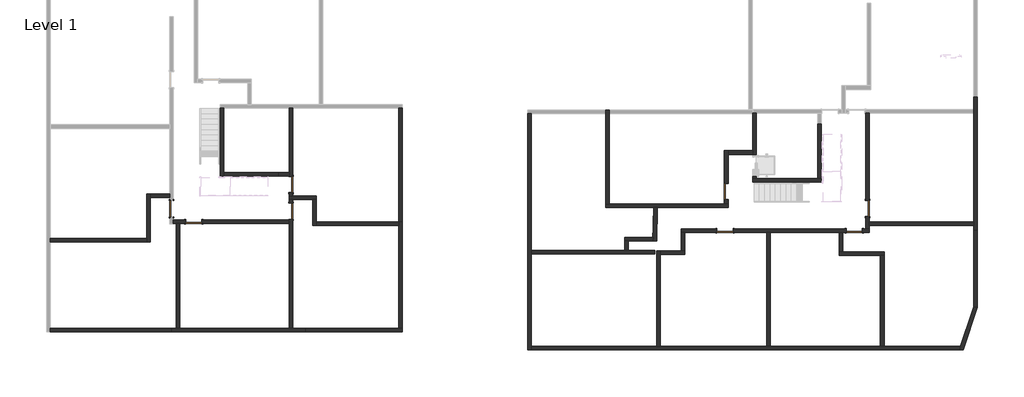
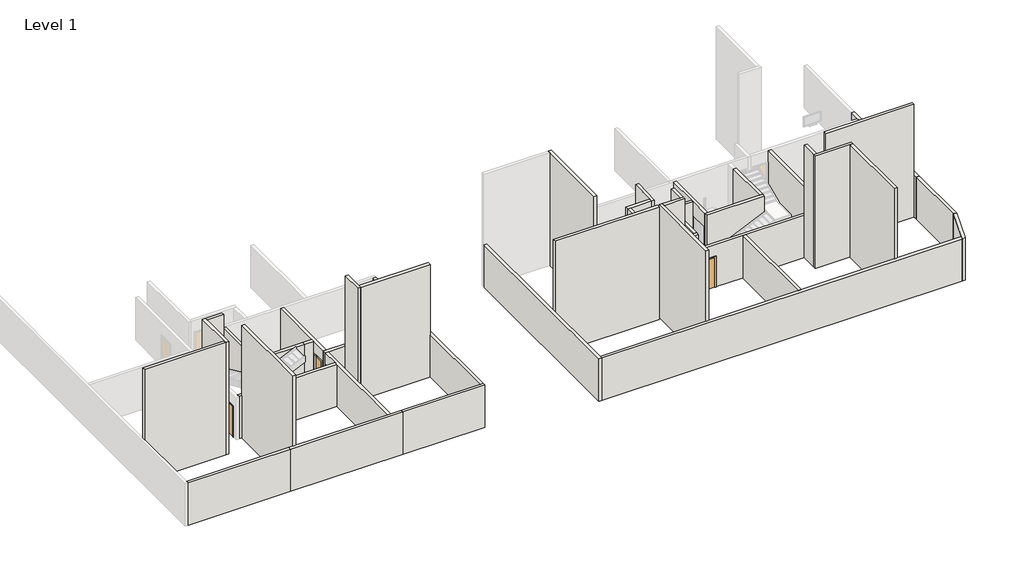
# One storey, part 1 of 2: 44 walls, 8 doors.
# Revit data of these elements (continued)
# Room, not placed, phase "New Construction", upper offset 0 cm, lower offset 0 cm
#   Number = "5"
#   Name = "Room"
# Room, not placed, phase "New Construction", upper offset 0 cm, lower offset 0 cm
#   Number = "6"
#   Name = "Room"
# Room at (-9476.825, 5160.6) mm, phase "New Construction", upper level "Level 1", upper offset 243.84 cm, lower offset 0 cm
#   Number = "124"
#   Name = "Room"
# Room, not placed, phase "New Construction", upper offset 0 cm, lower offset 0 cm
#   Number = "34"
#   Name = "Room"
# Room, not placed, phase "New Construction", upper offset 0 cm, lower offset 0 cm
#   Number = "35"
#   Name = "Room"
# Room, not placed, phase "New Construction", upper offset 0 cm, lower offset 0 cm
#   Number = "9"
#   Name = "Room"
# Room, not placed, phase "New Construction", upper offset 0 cm, lower offset 0 cm
#   Number = "10"
#   Name = "Room"
# Room, not placed, phase "New Construction", upper offset 0 cm, lower offset 0 cm
#   Number = "125"
#   Name = "Room"
# Room, not placed, phase "New Construction", upper offset 0 cm, lower offset 0 cm
#   Number = "126"
#   Name = "Room"
# Room, not placed, phase "New Construction", upper offset 0 cm, lower offset 0 cm
#   Number = "127"
#   Name = "Room"
# Room, not placed, phase "New Construction", upper offset 0 cm, lower offset 0 cm
#   Number = "128"
#   Name = "Room"
# Room, not placed, phase "New Construction", upper offset 0 cm, lower offset 0 cm
#   Number = "129"
#   Name = "Room"
# Room, not placed, phase "New Construction", upper offset 0 cm, lower offset 0 cm
#   Number = "91"
#   Name = "Room"
# Room at (-20321.225, 11202.195) mm, phase "New Construction", upper level "Level 1", upper offset 243.84 cm, lower offset 0 cm
#   Number = "130"
#   Name = "Room"
# Room at (-5594.466, -7580.79) mm, phase "New Construction", upper level "Level 1", upper offset 243.84 cm, lower offset 0 cm
#   Number = "131"
#   Name = "Room"
# Room at (-4954.966, -1430.614) mm, phase "New Construction", upper level "Level 1", upper offset 243.84 cm, lower offset 0 cm
#   Number = "132"
#   Name = "Room"
# Room at (-12237.947, 10302.814) mm, phase "New Construction", upper level "Level 1", upper offset 243.84 cm, lower offset 0 cm
#   Number = "133"
#   Name = "Room"
# Room, not placed, phase "New Construction", upper offset 0 cm, lower offset 0 cm
#   Number = ""
#   Name = ""
# Room, not placed, phase "New Construction", upper offset 0 cm, lower offset 0 cm
#   Number = "70"
#   Name = "Room"
# Room, not placed, phase "New Construction", upper offset 0 cm, lower offset 0 cm
#   Number = "71"
#   Name = "Room"
# Room, not placed, phase "New Construction", upper offset 0 cm, lower offset 0 cm
#   Number = "92"
#   Name = "Room"
# Room, not placed, phase "New Construction", upper offset 0 cm, lower offset 0 cm
#   Number = ""
#   Name = ""
# Room, not placed, phase "New Construction", upper offset 0 cm, lower offset 0 cm
#   Number = ""
#   Name = ""
# Room, not placed, phase "New Construction", upper offset 0 cm, lower offset 0 cm
#   Number = "37"
#   Name = "Room"
# Room, not placed, phase "New Construction", upper offset 0 cm, lower offset 0 cm
#   Number = ""
#   Name = "Banyo"
# Room, not placed, phase "New Construction", upper offset 0 cm, lower offset 0 cm
#   Number = ""
#   Name = ""
# Room, not placed, phase "New Construction", upper offset 0 cm, lower offset 0 cm
#   Number = ""
#   Name = "Yatak Odası"
# Room, not placed, phase "New Construction", upper offset 0 cm, lower offset 0 cm
#   Number = "39"
#   Name = "Room"
# Room, not placed, phase "New Construction", upper offset 0 cm, lower offset 0 cm
#   Number = ""
#   Name = "Salon-Mutfak"
# Area at (-11214.009, 13625.616) mm, upper offset 243.84 cm, lower offset 0 cm
#   Number = "9"
#   Name = "Area"
# Room, not placed, phase "New Construction", upper offset 0 cm, lower offset 0 cm
#   Number = "134"
#   Name = "Room"
# Room at (-19334.034, -2481.955) mm, phase "New Construction", upper level "Level 1", upper offset 243.84 cm, lower offset 0 cm
#   Number = "135"
#   Name = "Room"
# Room, not placed, phase "New Construction", upper offset 0 cm, lower offset 0 cm
#   Number = "40"
#   Name = "Room"
# Room, not placed, phase "New Construction", upper offset 0 cm, lower offset 0 cm
#   Number = "41"
#   Name = "Room"
# Area, not placed, upper offset 0 cm, lower offset 0 cm
#   Number = "8"
#   Name = "Dere Parsel Toplam Alan"
# Room, not placed, phase "New Construction", upper offset 0 cm, lower offset 0 cm
#   Number = "108"
#   Name = "ASANSÖR"
# Room, not placed, phase "New Construction", upper offset 0 cm, lower offset 0 cm
#   Number = "89"
#   Name = "Room"
# Room, not placed, phase "New Construction", upper offset 0 cm, lower offset 0 cm
#   Number = "19"
#   Name = "Room"
# Room, not placed, phase "New Construction", upper offset 0 cm, lower offset 0 cm
#   Number = ""
#   Name = ""
# Room, not placed, phase "New Construction", upper offset 0 cm, lower offset 0 cm
#   Number = "21"
#   Name = "Room"
# Room, not placed, phase "New Construction", upper offset 0 cm, lower offset 0 cm
#   Number = "22"
#   Name = "Room"
# Room, not placed, phase "New Construction", upper offset 0 cm, lower offset 0 cm
#   Number = "23"
#   Name = "Room"
# Room, not placed, phase "New Construction", upper offset 0 cm, lower offset 0 cm
#   Number = "24"
#   Name = "Room"
# Room, not placed, phase "New Construction", upper offset 0 cm, lower offset 0 cm
#   Number = "25"
#   Name = "Room"
# Room, not placed, phase "New Construction", upper offset 0 cm, lower offset 0 cm
#   Number = "64"
#   Name = "Room"
# Room, not placed, phase "New Construction", upper offset 0 cm, lower offset 0 cm
#   Number = "65"
#   Name = "Room"
# Room, not placed, phase "New Construction", upper offset 0 cm, lower offset 0 cm
#   Number = "66"
#   Name = "Room"
# Room, not placed, phase "New Construction", upper offset 0 cm, lower offset 0 cm
#   Number = ""
#   Name = ""
# Room, not placed, phase "New Construction", upper offset 0 cm, lower offset 0 cm
#   Number = "27"
#   Name = "Room"
# Room, not placed, phase "New Construction", upper offset 0 cm, lower offset 0 cm
#   Number = "42"
#   Name = "Room"
# Area, not placed, upper offset 0 cm, lower offset 0 cm
#   Number = "2"
#   Name = "Area"
# Room, not placed, phase "New Construction", upper offset 0 cm, lower offset 0 cm
#   Number = "43"
#   Name = "Room"
# Room, not placed, phase "New Construction", upper offset 0 cm, lower offset 0 cm
#   Number = ""
#   Name = ""
# Room, not placed, phase "New Construction", upper offset 0 cm, lower offset 0 cm
#   Number = "94"
#   Name = "Room"
# Room, not placed, phase "New Construction", upper offset 0 cm, lower offset 0 cm
#   Number = ""
#   Name = ""
# Room at (-18935.383, 3898.657) mm, phase "New Construction", upper level "Level 1", upper offset 243.84 cm, lower offset 0 cm
#   Number = "136"
#   Name = "Room"
# Room, not placed, phase "New Construction", upper offset 0 cm, lower offset 0 cm
#   Number = "1"
#   Name = "Room"
# Area, not placed, upper offset 0 cm, lower offset 0 cm
#   Number = "3"
#   Name = "Area"
# Room, not placed, phase "New Construction", upper offset 0 cm, lower offset 0 cm
#   Number = "7"
#   Name = "Room"
# Room, not placed, phase "New Construction", upper offset 0 cm, lower offset 0 cm
#   Number = "8"
#   Name = "Room"
# Room, not placed, phase "New Construction", upper offset 0 cm, lower offset 0 cm
#   Number = "2"
#   Name = "Room"
# Room, not placed, phase "New Construction", upper offset 0 cm, lower offset 0 cm
#   Number = "46"
#   Name = "Room"
# Room, not placed, phase "New Construction", upper offset 0 cm, lower offset 0 cm
#   Number = "3"
#   Name = "Room"
# Room, not placed, phase "New Construction", upper offset 0 cm, lower offset 0 cm
#   Number = ""
#   Name = ""
# Room, not placed, phase "New Construction", upper offset 0 cm, lower offset 0 cm
#   Number = "4"
#   Name = "Room"
# Area, not placed, upper offset 0 cm, lower offset 0 cm
#   Number = "1"
#   Name = "Area"
# Room, not placed, phase "New Construction", upper offset 0 cm, lower offset 0 cm
#   Number = ""
#   Name = ""
# Room, not placed, phase "New Construction", upper offset 0 cm, lower offset 0 cm
#   Number = "29"
#   Name = "Room"
# Area, not placed, upper offset 0 cm, lower offset 0 cm
#   Number = "7"
#   Name = "Dere Parsel Toplam Alan"
# Room, not placed, phase "New Construction", upper offset 0 cm, lower offset 0 cm
#   Number = "95"
#   Name = "ASANSÖR"
# Room, not placed, phase "New Construction", upper offset 0 cm, lower offset 0 cm
#   Number = "96"
#   Name = "Room"
# Room, not placed, phase "New Construction", upper offset 0 cm, lower offset 0 cm
#   Number = "97"
#   Name = "7"
# Room, not placed, phase "New Construction", upper offset 0 cm, lower offset 0 cm
#   Number = "98"
#   Name = "8"
# Room, not placed, phase "New Construction", upper offset 0 cm, lower offset 0 cm
#   Number = "99"
#   Name = "9"
# Room, not placed, phase "New Construction", upper offset 0 cm, lower offset 0 cm
#   Number = "100"
#   Name = "1"
# Room, not placed, phase "New Construction", upper offset 0 cm, lower offset 0 cm
#   Number = "101"
#   Name = "5"
# Room, not placed, phase "New Construction", upper offset 0 cm, lower offset 0 cm
#   Number = "102"
#   Name = "2"
# Room, not placed, phase "New Construction", upper offset 0 cm, lower offset 0 cm
#   Number = "103"
#   Name = "4"
# Room, not placed, phase "New Construction", upper offset 0 cm, lower offset 0 cm
#   Number = "104"
#   Name = "3"
# Room, not placed, phase "New Construction", upper offset 0 cm, lower offset 0 cm
#   Number = "105"
#   Name = "6"
